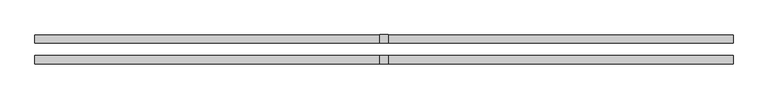
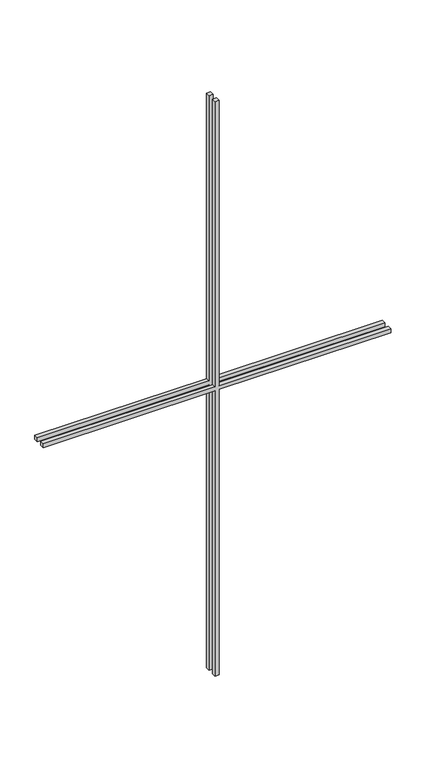
"""IFC4 building model written with IfcOpenShell, lengths in millimetres: proxy geometry, M_Padrão do montante_2x2 : M_Padrão do montante_2x2."""

import ifcopenshell
import ifcopenshell.guid

model = None  # the IFC model being written
_history = None  # IfcOwnerHistory: only IFC2X3 demands one
_inside = {}  # id of a spatial element -> (the spatial element, [elements in it])
_under = {}  # id of a project, library or spatial element -> (it, [spatial elements below it])
_declared = {}  # id of a project -> (the project, [libraries it declares])
_typed = {}  # id of a type object -> (the type object, [elements of that type])
_made_of = {}  # id of a material, layer set ... -> (it, [elements and type objects made of it])


def new_model(schema):
    """Start an empty IFC model of exactly this schema.

    Asked for "IFC4X3", IfcOpenShell would pick the latest addendum, in which some entities
    have other attributes; the version numbers below select the first issue.
    IFC2X3 requires an IfcOwnerHistory on every rooted entity: one is made here for all.
    """
    global model, _history
    if schema == "IFC4X3":
        model = ifcopenshell.file(schema_version=(4, 3, 0, 0))
    else:
        model = ifcopenshell.file(schema=schema)
    _inside.clear()
    _under.clear()
    _declared.clear()
    _typed.clear()
    _made_of.clear()
    _history = None
    if model.schema == "IFC2X3":
        org = make("IfcOrganization", Name="unknown")
        user = make(
            "IfcPersonAndOrganization",
            ThePerson=make("IfcPerson", FamilyName="unknown"),
            TheOrganization=org,
        )
        app = make(
            "IfcApplication",
            ApplicationDeveloper=org,
            Version="unknown",
            ApplicationFullName="unknown",
            ApplicationIdentifier="unknown",
        )
        _history = make(
            "IfcOwnerHistory",
            OwningUser=user,
            OwningApplication=app,
            ChangeAction="ADDED",
            CreationDate=0,
        )
    return model


def make(cls, **values):
    """One entity of the class cls with the attributes given. An attribute that is None is left unset."""
    return model.create_entity(
        cls, **{name: value for name, value in values.items() if value is not None}
    )


def rooted(cls, **values):
    """An entity with a GlobalId (a new one), such as an element, a storey or a relation."""
    return make(cls, GlobalId=ifcopenshell.guid.new(), OwnerHistory=_history, **values)


def si_unit(unit_type, name, prefix=None):
    """IfcSIUnit, for example si_unit("LENGTHUNIT", "METRE", prefix="MILLI")."""
    return make("IfcSIUnit", UnitType=unit_type, Prefix=prefix, Name=name)


def assignment(units):
    """IfcUnitAssignment: the units of a project."""
    return None if units is None else make("IfcUnitAssignment", Units=units)


def point(xyz):
    """IfcCartesianPoint."""
    return None if xyz is None else make("IfcCartesianPoint", Coordinates=xyz)


def direction(xyz):
    """IfcDirection."""
    return None if xyz is None else make("IfcDirection", DirectionRatios=xyz)


def frame(location, z_axis=None, x_axis=None):
    """IfcAxis2Placement3D, a coordinate frame: its origin and axes. An axis left out is left unset."""
    return make(
        "IfcAxis2Placement3D",
        Location=point(location),
        Axis=direction(z_axis),
        RefDirection=direction(x_axis),
    )


def origin():
    """The frame at (0, 0, 0) with its axes left unset."""
    return frame((0.0, 0.0, 0.0))


def place(relative_to, where):
    """IfcLocalPlacement: puts the frame where relative to a parent placement (None: the world)."""
    return make(
        "IfcLocalPlacement", PlacementRelTo=relative_to, RelativePlacement=where
    )


def context(
    kind, dimensions, precision=None, world=None, true_north=None, identifier=None
):
    """IfcGeometricRepresentationContext, for example the 3D "Model" context."""
    return make(
        "IfcGeometricRepresentationContext",
        ContextIdentifier=identifier,
        ContextType=kind,
        CoordinateSpaceDimension=dimensions,
        Precision=precision,
        WorldCoordinateSystem=world,
        TrueNorth=true_north,
    )


def project(units=None, contexts=None):
    """IfcProject with its units and contexts."""
    return rooted(
        "IfcProject",
        Name="project",
        RepresentationContexts=contexts,
        UnitsInContext=assignment(units),
    )


def spatial(cls, under=None, at=None, **own):
    """A site, building, storey or space (cls), placed at a placement, below another one or the project."""
    s = rooted(cls, ObjectPlacement=at, **own)
    if under is not None:
        _under.setdefault(under.id(), (under, []))[1].append(s)
    return s


def polyline(points):
    """IfcPolyline through the points."""
    return make("IfcPolyline", Points=[point(p) for p in points])


def outline(outer, holes=None, kind="AREA"):
    """IfcArbitraryClosedProfileDef: a profile drawn as a closed curve; with holes, ...WithVoids."""
    if holes is None:
        return make("IfcArbitraryClosedProfileDef", ProfileType=kind, OuterCurve=outer)
    return make(
        "IfcArbitraryProfileDefWithVoids",
        ProfileType=kind,
        OuterCurve=outer,
        InnerCurves=holes,
    )


def extrude(swept, where, along, depth):
    """IfcExtrudedAreaSolid: the profile swept, set in the frame where, extruded along a direction by depth."""
    return make(
        "IfcExtrudedAreaSolid",
        SweptArea=swept,
        Position=where,
        ExtrudedDirection=direction(along),
        Depth=depth,
    )


def shape(context_of_items, identifier, shape_type, items):
    """IfcShapeRepresentation: the items that make up one representation, for example the "Body"."""
    return make(
        "IfcShapeRepresentation",
        ContextOfItems=context_of_items,
        RepresentationIdentifier=identifier,
        RepresentationType=shape_type,
        Items=items,
    )


def source(mapping_origin, context_of_items, identifier, shape_type, items):
    """IfcRepresentationMap: a shape defined once, which mapped items show again and again."""
    return make(
        "IfcRepresentationMap",
        MappingOrigin=mapping_origin,
        MappedRepresentation=shape(context_of_items, identifier, shape_type, items),
    )


def transform(
    local_origin,
    x_axis=None,
    y_axis=None,
    z_axis=None,
    scale=None,
    scale2=None,
    scale3=None,
    uniform=True,
):
    """IfcCartesianTransformationOperator3D, or its non-uniform kind. x_axis, y_axis, z_axis: its Axis1, 2, 3."""
    if uniform:
        return make(
            "IfcCartesianTransformationOperator3D",
            Axis1=direction(x_axis),
            Axis2=direction(y_axis),
            LocalOrigin=point(local_origin),
            Scale=scale,
            Axis3=direction(z_axis),
        )
    return make(
        "IfcCartesianTransformationOperator3DnonUniform",
        Axis1=direction(x_axis),
        Axis2=direction(y_axis),
        LocalOrigin=point(local_origin),
        Scale=scale,
        Axis3=direction(z_axis),
        Scale2=scale2,
        Scale3=scale3,
    )


def mapped(mapping_source, mapping_target):
    """IfcMappedItem: shows the shape of a source again, moved by a transform."""
    return make(
        "IfcMappedItem", MappingSource=mapping_source, MappingTarget=mapping_target
    )


def made_of(thing, what):
    """Note that an element or type object is made of a material, layer set ...; save() writes the relation."""
    if what is not None:
        _made_of.setdefault(what.id(), (what, []))[1].append(thing)
    return thing


def element(
    cls,
    number,
    at=None,
    inside=None,
    cuts=None,
    type_object=None,
    material=None,
    context=None,
    identifier="Body",
    shape_type=None,
    held_by="IfcProductDefinitionShape",
    body=None,
    shapes=None,
    **own,
):
    """One element of the class cls, such as IfcWall. Its Tag is "e" and its number.

    at: its placement. inside: the storey or other place that contains it. cuts: it is an
    opening in that element (IfcRelVoidsElement). A single representation is given by context,
    identifier, shape_type and body (its items); several are given by shapes. held_by: the class
    of the entity that holds the representations. save() writes the other relations.
    """
    e = rooted(cls, Tag="e%d" % number, ObjectPlacement=at, **own)
    if body is not None:
        shapes = [shape(context, identifier, shape_type, body)]
    if shapes is not None:
        e.Representation = make(held_by, Representations=shapes)
    if inside is not None:
        _inside.setdefault(inside.id(), (inside, []))[1].append(e)
    if cuts is not None:
        rooted(
            "IfcRelVoidsElement", RelatingBuildingElement=cuts, RelatedOpeningElement=e
        )
    if type_object is not None:
        _typed.setdefault(type_object.id(), (type_object, []))[1].append(e)
    return made_of(e, material)


def aggregate(whole, parts):
    """IfcRelAggregates: a whole, such as a stair, and the parts it consists of."""
    return rooted("IfcRelAggregates", RelatingObject=whole, RelatedObjects=parts)


def save(model, path):
    """Write the relations noted so far, then the file.

    IfcRelAggregates (storeys below a building ...), IfcRelContainedInSpatialStructure (elements
    in a storey), IfcRelDefinesByType, IfcRelAssociatesMaterial and IfcRelDeclares: one each for
    every whole, place, type object, material and project.
    """
    for whole, parts in _under.values():
        aggregate(whole, parts)
    for where, things in _inside.values():
        rooted(
            "IfcRelContainedInSpatialStructure",
            RelatedElements=things,
            RelatingStructure=where,
        )
    for kind, things in _typed.values():
        rooted("IfcRelDefinesByType", RelatedObjects=things, RelatingType=kind)
    for what, things in _made_of.values():
        rooted("IfcRelAssociatesMaterial", RelatedObjects=things, RelatingMaterial=what)
    for by, libraries in _declared.values():
        rooted("IfcRelDeclares", RelatingContext=by, RelatedDefinitions=libraries)
    model.write(path)


def generic_models_776d06b5(model_context):
    return source(origin(), model_context, "Body", "SweptSolid", [
        extrude(outline(polyline([(933.325, -6.35), (933.325, -530.65), (920.625, -530.65), (920.625, -6.35), (0.0, -6.35), (0.0, 6.35), (920.625, 6.35), (920.625, 530.65), (933.325, 530.65), (933.325, 6.35), (1853.95, 6.35), (1853.95, -6.35), (933.325, -6.35)])), frame((0.0, 9.525, 0.0), z_axis=(0.0, 1.0, 0.0), x_axis=(0.0, 0.0, 1.0)), (0.0, 0.0, 1.0), 12.7),
        extrude(outline(polyline([(933.325, -6.35), (933.325, -530.65), (920.625, -530.65), (920.625, -6.35), (0.0, -6.35), (0.0, 6.35), (920.625, 6.35), (920.625, 530.65), (933.325, 530.65), (933.325, 6.35), (1853.95, 6.35), (1853.95, -6.35), (933.325, -6.35)])), frame((0.0, -22.225, 0.0), z_axis=(0.0, 1.0, 0.0), x_axis=(0.0, 0.0, 1.0)), (0.0, 0.0, 1.0), 12.7),
    ])


if __name__ == "__main__":
    model = new_model("IFC4")
    model_context = context("Model", 3, world=origin())
    ifc_project = project(units=[si_unit("LENGTHUNIT", "METRE", prefix="MILLI")], contexts=[model_context])
    site = spatial("IfcSite", under=ifc_project)
    building = spatial("IfcBuilding", under=site)
    placement = place(None, origin())
    generic_models_shape = generic_models_776d06b5(model_context)
    element("IfcBuildingElementProxy", 1, Name="M_Padrão do montante_2x2 : M_Padrão do montante_2x2", ObjectType="M_Padrão do montante_2x2 : M_Padrão do montante_2x2", at=placement, inside=building, context=model_context, shape_type="MappedRepresentation", body=[
        mapped(generic_models_shape, transform((0.0, 0.0, 0.0), x_axis=(1.0, 0.0, 0.0), y_axis=(0.0, 1.0, 0.0), z_axis=(0.0, 0.0, 1.0))),
    ])
    save(model, "model.ifc")

# Revit data of these elements
# Type "M_Padrão do montante_2x2 : M_Padrão do montante_2x2"
#   Largura [instance default] = 1.200 m
#   Espessura = 0.0127 m
#   Altura [instance default] = 1.200 m
#   Distância = 0.01905 m
#   Material interior [instance default] = none
#   Material externo [instance default] = none
#   Default Elevation = 0
# Element 1 (IfcBuildingElementProxy, "M_Padrão do montante_2x2 : M_Padrão do montante_2x2")
#   Largura = 1.0613 m
#   Altura = 1.85395 m
#   Material interior = Madeira – Manchada
#   Material externo = Revestimento – Branco
#   Materials on its faces: "Revestimento – Branco", "Madeira – Manchada"
# Materials
#   "Revestimento – Branco": class "Madeira", colour RGB 242 242 238, transparency 0, Cost = 0
#   "Madeira – Manchada": class "Madeira", colour RGB 224 178 126, transparency 0, Cost = 0
